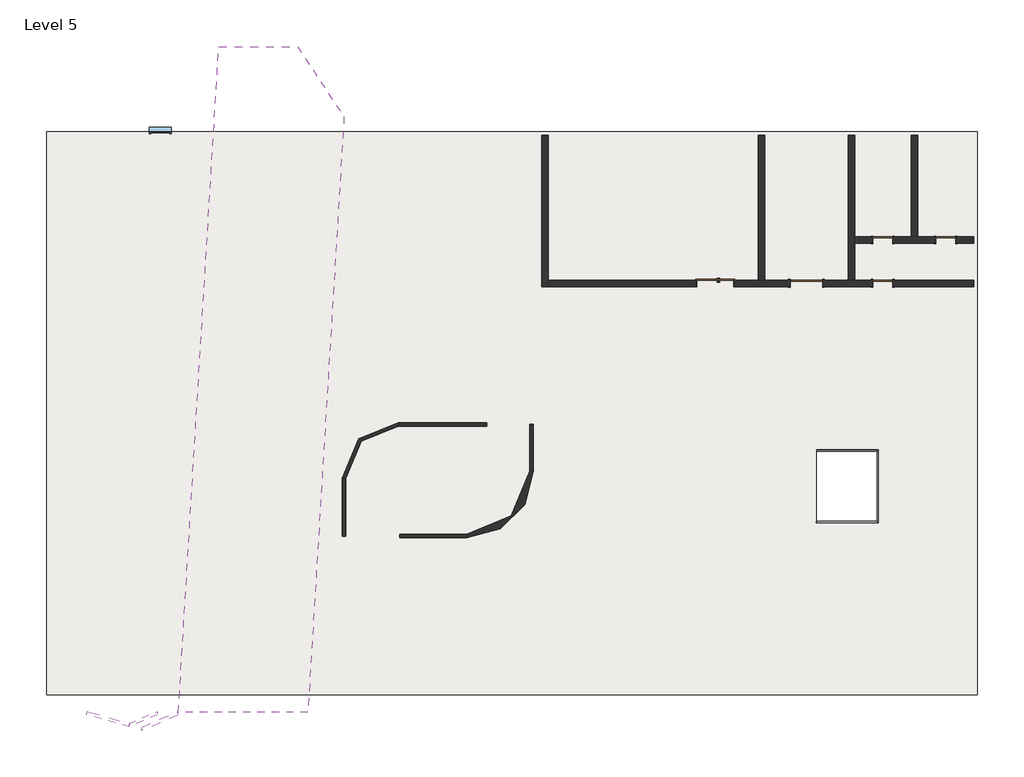
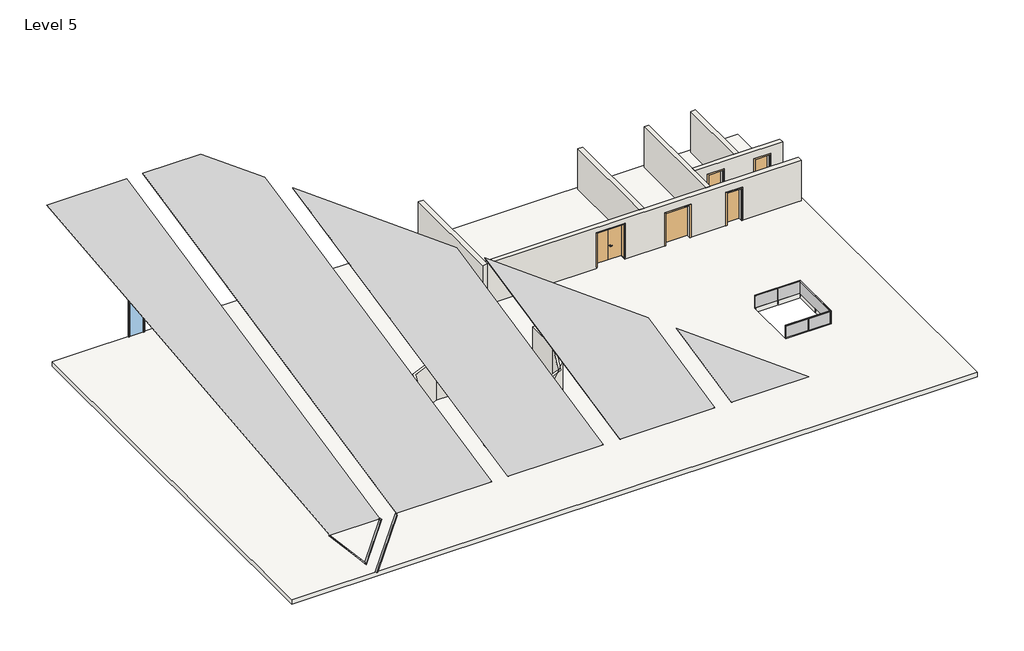
# One storey: 12 walls, 5 doors, 3 members, 1 plate, 1 railing, 1 slab, 1 window.
"""IFC4 building model written with IfcOpenShell, lengths in millimetres."""

import ifcopenshell
import ifcopenshell.guid

model = None  # the IFC model being written
_history = None  # IfcOwnerHistory: only IFC2X3 demands one
_inside = {}  # id of a spatial element -> (the spatial element, [elements in it])
_under = {}  # id of a project, library or spatial element -> (it, [spatial elements below it])
_declared = {}  # id of a project -> (the project, [libraries it declares])
_typed = {}  # id of a type object -> (the type object, [elements of that type])
_made_of = {}  # id of a material, layer set ... -> (it, [elements and type objects made of it])


def new_model(schema):
    """Start an empty IFC model of exactly this schema.

    Asked for "IFC4X3", IfcOpenShell would pick the latest addendum, in which some entities
    have other attributes; the version numbers below select the first issue.
    IFC2X3 requires an IfcOwnerHistory on every rooted entity: one is made here for all.
    """
    global model, _history
    if schema == "IFC4X3":
        model = ifcopenshell.file(schema_version=(4, 3, 0, 0))
    else:
        model = ifcopenshell.file(schema=schema)
    _inside.clear()
    _under.clear()
    _declared.clear()
    _typed.clear()
    _made_of.clear()
    _history = None
    if model.schema == "IFC2X3":
        org = make("IfcOrganization", Name="unknown")
        user = make(
            "IfcPersonAndOrganization",
            ThePerson=make("IfcPerson", FamilyName="unknown"),
            TheOrganization=org,
        )
        app = make(
            "IfcApplication",
            ApplicationDeveloper=org,
            Version="unknown",
            ApplicationFullName="unknown",
            ApplicationIdentifier="unknown",
        )
        _history = make(
            "IfcOwnerHistory",
            OwningUser=user,
            OwningApplication=app,
            ChangeAction="ADDED",
            CreationDate=0,
        )
    return model


def make(cls, **values):
    """One entity of the class cls with the attributes given. An attribute that is None is left unset."""
    return model.create_entity(
        cls, **{name: value for name, value in values.items() if value is not None}
    )


def rooted(cls, **values):
    """An entity with a GlobalId (a new one), such as an element, a storey or a relation."""
    return make(cls, GlobalId=ifcopenshell.guid.new(), OwnerHistory=_history, **values)


def si_unit(unit_type, name, prefix=None):
    """IfcSIUnit, for example si_unit("LENGTHUNIT", "METRE", prefix="MILLI")."""
    return make("IfcSIUnit", UnitType=unit_type, Prefix=prefix, Name=name)


def assignment(units):
    """IfcUnitAssignment: the units of a project."""
    return None if units is None else make("IfcUnitAssignment", Units=units)


def point(xyz):
    """IfcCartesianPoint."""
    return None if xyz is None else make("IfcCartesianPoint", Coordinates=xyz)


def direction(xyz):
    """IfcDirection."""
    return None if xyz is None else make("IfcDirection", DirectionRatios=xyz)


def frame(location, z_axis=None, x_axis=None):
    """IfcAxis2Placement3D, a coordinate frame: its origin and axes. An axis left out is left unset."""
    return make(
        "IfcAxis2Placement3D",
        Location=point(location),
        Axis=direction(z_axis),
        RefDirection=direction(x_axis),
    )


def frame_2d(location, x_axis=None):
    """IfcAxis2Placement2D, a coordinate frame in the plane: its origin and x axis."""
    return make(
        "IfcAxis2Placement2D", Location=point(location), RefDirection=direction(x_axis)
    )


def origin():
    """The frame at (0, 0, 0) with its axes left unset."""
    return frame((0.0, 0.0, 0.0))


def origin_with_axes():
    """The frame at (0, 0, 0) with the z axis (0, 0, 1) and the x axis (1, 0, 0) written out."""
    return frame((0.0, 0.0, 0.0), z_axis=(0.0, 0.0, 1.0), x_axis=(1.0, 0.0, 0.0))


def place(relative_to, where):
    """IfcLocalPlacement: puts the frame where relative to a parent placement (None: the world)."""
    return make(
        "IfcLocalPlacement", PlacementRelTo=relative_to, RelativePlacement=where
    )


def context(
    kind, dimensions, precision=None, world=None, true_north=None, identifier=None
):
    """IfcGeometricRepresentationContext, for example the 3D "Model" context."""
    return make(
        "IfcGeometricRepresentationContext",
        ContextIdentifier=identifier,
        ContextType=kind,
        CoordinateSpaceDimension=dimensions,
        Precision=precision,
        WorldCoordinateSystem=world,
        TrueNorth=true_north,
    )


def project(units=None, contexts=None):
    """IfcProject with its units and contexts."""
    return rooted(
        "IfcProject",
        Name="project",
        RepresentationContexts=contexts,
        UnitsInContext=assignment(units),
    )


def spatial(cls, under=None, at=None, **own):
    """A site, building, storey or space (cls), placed at a placement, below another one or the project."""
    s = rooted(cls, ObjectPlacement=at, **own)
    if under is not None:
        _under.setdefault(under.id(), (under, []))[1].append(s)
    return s


def polyline(points):
    """IfcPolyline through the points."""
    return make("IfcPolyline", Points=[point(p) for p in points])


def circle_curve(where, radius):
    """IfcCircle in the frame where."""
    return make("IfcCircle", Position=where, Radius=radius)


def ellipse_curve(where, semi_axis1, semi_axis2):
    """IfcEllipse in the frame where."""
    return make(
        "IfcEllipse", Position=where, SemiAxis1=semi_axis1, SemiAxis2=semi_axis2
    )


def trimmed(basis, trim1, trim2, sense, master):
    """IfcTrimmedCurve: the piece of a basis curve between two trims."""
    return make(
        "IfcTrimmedCurve",
        BasisCurve=basis,
        Trim1=trim1,
        Trim2=trim2,
        SenseAgreement=sense,
        MasterRepresentation=master,
    )


def segment(curve, same_sense, transition):
    """IfcCompositeCurveSegment."""
    return make(
        "IfcCompositeCurveSegment",
        Transition=transition,
        SameSense=same_sense,
        ParentCurve=curve,
    )


def composite_curve(segments, self_intersect=None):
    """IfcCompositeCurve: segments joined end to end."""
    return make("IfcCompositeCurve", Segments=segments, SelfIntersect=self_intersect)


def outline(outer, holes=None, kind="AREA"):
    """IfcArbitraryClosedProfileDef: a profile drawn as a closed curve; with holes, ...WithVoids."""
    if holes is None:
        return make("IfcArbitraryClosedProfileDef", ProfileType=kind, OuterCurve=outer)
    return make(
        "IfcArbitraryProfileDefWithVoids",
        ProfileType=kind,
        OuterCurve=outer,
        InnerCurves=holes,
    )


def extrude(swept, where, along, depth):
    """IfcExtrudedAreaSolid: the profile swept, set in the frame where, extruded along a direction by depth."""
    return make(
        "IfcExtrudedAreaSolid",
        SweptArea=swept,
        Position=where,
        ExtrudedDirection=direction(along),
        Depth=depth,
    )


def faces_of(points, faces, orient=None, outer=None):
    """IfcFace entities. A face is a list of loops; a loop is a list of indices into points, from 0.

    orient and outer hold one flag for each loop. By default every Orientation is true, the
    first loop of a face is its IfcFaceOuterBound and the others are IfcFaceBound.
    """
    made = []
    for i, loops in enumerate(faces):
        bounds = []
        for j, loop in enumerate(loops):
            is_outer = j == 0 if outer is None else outer[i][j]
            bounds.append(
                make(
                    "IfcFaceOuterBound" if is_outer else "IfcFaceBound",
                    Bound=make("IfcPolyLoop", Polygon=[points[k] for k in loop]),
                    Orientation=True if orient is None else orient[i][j],
                )
            )
        made.append(make("IfcFace", Bounds=bounds))
    return made


def faceted_brep(points, faces, orient=None, outer=None, voids=None):
    """IfcFacetedBrep: a solid bounded by flat faces; with voids (closed shells), ...WithVoids."""
    shared = [point(p) for p in points]
    hull = make("IfcClosedShell", CfsFaces=faces_of(shared, faces, orient, outer))
    if voids is None:
        return make("IfcFacetedBrep", Outer=hull)
    return make(
        "IfcFacetedBrepWithVoids",
        Outer=hull,
        Voids=[
            make(cls, CfsFaces=faces_of(shared, fs, o, b)) for cls, fs, o, b in voids
        ],
    )


def shape(context_of_items, identifier, shape_type, items):
    """IfcShapeRepresentation: the items that make up one representation, for example the "Body"."""
    return make(
        "IfcShapeRepresentation",
        ContextOfItems=context_of_items,
        RepresentationIdentifier=identifier,
        RepresentationType=shape_type,
        Items=items,
    )


def source(mapping_origin, context_of_items, identifier, shape_type, items):
    """IfcRepresentationMap: a shape defined once, which mapped items show again and again."""
    return make(
        "IfcRepresentationMap",
        MappingOrigin=mapping_origin,
        MappedRepresentation=shape(context_of_items, identifier, shape_type, items),
    )


def transform(
    local_origin,
    x_axis=None,
    y_axis=None,
    z_axis=None,
    scale=None,
    scale2=None,
    scale3=None,
    uniform=True,
):
    """IfcCartesianTransformationOperator3D, or its non-uniform kind. x_axis, y_axis, z_axis: its Axis1, 2, 3."""
    if uniform:
        return make(
            "IfcCartesianTransformationOperator3D",
            Axis1=direction(x_axis),
            Axis2=direction(y_axis),
            LocalOrigin=point(local_origin),
            Scale=scale,
            Axis3=direction(z_axis),
        )
    return make(
        "IfcCartesianTransformationOperator3DnonUniform",
        Axis1=direction(x_axis),
        Axis2=direction(y_axis),
        LocalOrigin=point(local_origin),
        Scale=scale,
        Axis3=direction(z_axis),
        Scale2=scale2,
        Scale3=scale3,
    )


def mapped(mapping_source, mapping_target):
    """IfcMappedItem: shows the shape of a source again, moved by a transform."""
    return make(
        "IfcMappedItem", MappingSource=mapping_source, MappingTarget=mapping_target
    )


def made_of(thing, what):
    """Note that an element or type object is made of a material, layer set ...; save() writes the relation."""
    if what is not None:
        _made_of.setdefault(what.id(), (what, []))[1].append(thing)
    return thing


def element(
    cls,
    number,
    at=None,
    inside=None,
    cuts=None,
    type_object=None,
    material=None,
    context=None,
    identifier="Body",
    shape_type=None,
    held_by="IfcProductDefinitionShape",
    body=None,
    shapes=None,
    **own,
):
    """One element of the class cls, such as IfcWall. Its Tag is "e" and its number.

    at: its placement. inside: the storey or other place that contains it. cuts: it is an
    opening in that element (IfcRelVoidsElement). A single representation is given by context,
    identifier, shape_type and body (its items); several are given by shapes. held_by: the class
    of the entity that holds the representations. save() writes the other relations.
    """
    e = rooted(cls, Tag="e%d" % number, ObjectPlacement=at, **own)
    if body is not None:
        shapes = [shape(context, identifier, shape_type, body)]
    if shapes is not None:
        e.Representation = make(held_by, Representations=shapes)
    if inside is not None:
        _inside.setdefault(inside.id(), (inside, []))[1].append(e)
    if cuts is not None:
        rooted(
            "IfcRelVoidsElement", RelatingBuildingElement=cuts, RelatedOpeningElement=e
        )
    if type_object is not None:
        _typed.setdefault(type_object.id(), (type_object, []))[1].append(e)
    return made_of(e, material)


def aggregate(whole, parts):
    """IfcRelAggregates: a whole, such as a stair, and the parts it consists of."""
    return rooted("IfcRelAggregates", RelatingObject=whole, RelatedObjects=parts)


def save(model, path):
    """Write the relations noted so far, then the file.

    IfcRelAggregates (storeys below a building ...), IfcRelContainedInSpatialStructure (elements
    in a storey), IfcRelDefinesByType, IfcRelAssociatesMaterial and IfcRelDeclares: one each for
    every whole, place, type object, material and project.
    """
    for whole, parts in _under.values():
        aggregate(whole, parts)
    for where, things in _inside.values():
        rooted(
            "IfcRelContainedInSpatialStructure",
            RelatedElements=things,
            RelatingStructure=where,
        )
    for kind, things in _typed.values():
        rooted("IfcRelDefinesByType", RelatedObjects=things, RelatingType=kind)
    for what, things in _made_of.values():
        rooted("IfcRelAssociatesMaterial", RelatedObjects=things, RelatingMaterial=what)
    for by, libraries in _declared.values():
        rooted("IfcRelDeclares", RelatingContext=by, RelatedDefinitions=libraries)
    model.write(path)


def plane_surface(at):
    """IfcPlane: the flat surface through the origin of the frame at, square to its z axis."""
    return make("IfcPlane", Position=at)


def cylinder_surface(at, radius):
    """IfcCylindricalSurface: all points at the distance radius from the z axis of the frame at."""
    return make("IfcCylindricalSurface", Position=at, Radius=radius)


def advanced_brep(points, edges, surfaces, faces):
    """IfcAdvancedBrep: a solid bounded by faces that lie on surfaces and meet in shared edges.

    An edge is (start, end): straight between two places in points (the first is 0);
    or (start, end, curve); or (start, end, curve, False) where it runs against its curve.
    A face is (place in surfaces, loops), or (place, loops, False) where it looks against
    its surface's normal. A loop lists edges by number (the first is 1), with a minus sign
    where the edge is run from its end to its start. The first loop is the outer one.
    """
    corners = [point(p) for p in points]
    vertices = [make("IfcVertexPoint", VertexGeometry=c) for c in corners]
    made = []
    for start, end, *more in edges:
        made.append(
            make(
                "IfcEdgeCurve",
                EdgeStart=vertices[start],
                EdgeEnd=vertices[end],
                EdgeGeometry=more[0] if more else make("IfcPolyline", Points=[corners[start], corners[end]]),
                SameSense=more[1] if len(more) > 1 else True,
            )
        )
    hull = []
    for where, loops, *sense in faces:
        bounds = []
        for j, loop in enumerate(loops):
            ring = [make("IfcOrientedEdge", EdgeElement=made[abs(k) - 1], Orientation=k > 0) for k in loop]
            bounds.append(
                make(
                    "IfcFaceOuterBound" if j == 0 else "IfcFaceBound",
                    Bound=make("IfcEdgeLoop", EdgeList=ring),
                    Orientation=True,
                )
            )
        hull.append(make("IfcAdvancedFace", Bounds=bounds, FaceSurface=surfaces[where], SameSense=sense[0] if sense else True))
    return make("IfcAdvancedBrep", Outer=make("IfcClosedShell", CfsFaces=hull))


def door_double_flush_variable_door_double_flush_variable_ac6c3b87(model_context):
    return source(origin(), model_context, "Body", "SolidModel", [
        advanced_brep(
        [(90.0, 139.4346141, 1000.0), (110.0, 139.4346141, 1000.0), (90.0, 69.4346141, 1000.0), (110.0, 89.4346141, 1000.0), (220.0, 69.4346141, 1000.0), (220.0, 89.4346141, 1000.0)],
        [
            (0, 1, circle_curve(frame((100.0, 139.4346141, 1000.0), z_axis=(0.0, 1.0, 0.0), x_axis=(1.0, 0.0, 0.0)), 10.0)),
            (1, 0, circle_curve(frame((100.0, 139.4346141, 1000.0), z_axis=(0.0, 1.0, 0.0), x_axis=(1.0, 0.0, 0.0)), 10.0)),
            (0, 2),
            (2, 3, ellipse_curve(frame((100.0, 79.4346141, 1000.0), z_axis=(-0.7071067811865385, 0.7071067811865565, 0.0), x_axis=(0.7071067811865563, 0.7071067811865386, 0.0)), 14.1421356, 10.0)),
            (3, 1),
            (3, 2, ellipse_curve(frame((100.0, 79.4346141, 1000.0), z_axis=(-0.7071067811865385, 0.7071067811865565, 0.0), x_axis=(0.7071067811865563, 0.7071067811865386, 0.0)), 14.1421356, 10.0)),
            (4, 5, circle_curve(frame((220.0, 79.4346141, 1000.0), z_axis=(1.0, 0.0, 0.0), x_axis=(0.0, 1.0, 0.0)), 10.0)),
            (5, 4, circle_curve(frame((220.0, 79.4346141, 1000.0), z_axis=(1.0, 0.0, 0.0), x_axis=(0.0, 1.0, 0.0)), 10.0)),
            (2, 4),
            (5, 3),
        ],
        [
            plane_surface(frame((100.0, 139.4346141, -287.7526403), z_axis=(0.0, 1.0, 0.0), x_axis=(0.0, 0.0, 1.0))),
            cylinder_surface(frame((100.0, 139.4346141, 1000.0), z_axis=(0.0, 1.0, 0.0), x_axis=(1.0, 0.0, 0.0)), 10.0),
            plane_surface(frame((220.0, 79.4346141, -287.7526403), z_axis=(1.0, 0.0, 0.0), x_axis=(0.0, 0.0, 1.0))),
            cylinder_surface(frame((100.0, 79.4346141, 1000.0), z_axis=(-1.0, 0.0, 0.0), x_axis=(0.0, 1.0, 0.0)), 10.0),
        ],
        [
            (0, [[1, 2]]),
            (1, [[-1, 3, 4, 5]]),
            (1, [[-2, -5, 6, -3]]),
            (2, [[7, 8]]),
            (3, [[-4, 9, -8, 10]]),
            (3, [[-6, -10, -7, -9]]),
        ],
    ),
        advanced_brep(
        [(110.0, 199.4346141, 1000.0), (90.0, 199.4346141, 1000.0), (110.0, 229.4346141, 1000.0), (90.0, 249.4346141, 1000.0), (220.0, 229.4346141, 1000.0), (220.0, 249.4346141, 1000.0)],
        [
            (0, 1, circle_curve(frame((100.0, 199.4346141, 1000.0), z_axis=(0.0, -1.0, 0.0), x_axis=(-1.0, 0.0, 0.0)), 10.0)),
            (1, 0, circle_curve(frame((100.0, 199.4346141, 1000.0), z_axis=(0.0, -1.0, 0.0), x_axis=(-1.0, 0.0, 0.0)), 10.0)),
            (0, 2),
            (2, 3, ellipse_curve(frame((100.0, 239.4346141, 1000.0), z_axis=(-0.7071067811865475, -0.7071067811865475, 0.0), x_axis=(0.7071067811865474, -0.7071067811865476, 0.0)), 14.1421356, 10.0)),
            (3, 1),
            (3, 2, ellipse_curve(frame((100.0, 239.4346141, 1000.0), z_axis=(-0.7071067811865475, -0.7071067811865475, 0.0), x_axis=(0.7071067811865474, -0.7071067811865476, 0.0)), 14.1421356, 10.0)),
            (4, 5, circle_curve(frame((220.0, 239.4346141, 1000.0), z_axis=(1.0, 0.0, 0.0), x_axis=(0.0, 1.0, 0.0)), 10.0)),
            (5, 4, circle_curve(frame((220.0, 239.4346141, 1000.0), z_axis=(1.0, 0.0, 0.0), x_axis=(0.0, 1.0, 0.0)), 10.0)),
            (2, 4),
            (5, 3),
        ],
        [
            plane_surface(frame((100.0, 199.4346141, -287.7526403), z_axis=(0.0, -1.0, 0.0), x_axis=(0.0, 0.0, 1.0))),
            cylinder_surface(frame((100.0, 199.4346141, 1000.0), z_axis=(0.0, -1.0, 0.0), x_axis=(-1.0, 0.0, 0.0)), 10.0),
            plane_surface(frame((220.0, 239.4346141, -287.7526403), z_axis=(1.0, 0.0, 0.0), x_axis=(0.0, 0.0, 1.0))),
            cylinder_surface(frame((100.0, 239.4346141, 1000.0), z_axis=(-1.0, 0.0, 0.0), x_axis=(0.0, 1.0, 0.0)), 10.0),
        ],
        [
            (0, [[1, 2]]),
            (1, [[-1, 3, 4, 5]]),
            (1, [[-2, -5, 6, -3]]),
            (2, [[7, 8]]),
            (3, [[-4, 9, -8, 10]]),
            (3, [[-6, -10, -7, -9]]),
        ],
    ),
        extrude(outline(composite_curve([segment(trimmed(circle_curve(frame_2d((1000.0, 100.0)), 20.0), [point((1000.0, 80.0))], [point((1000.0, 120.0))], False, "CARTESIAN"), True, "CONTINUOUS"), segment(trimmed(circle_curve(frame_2d((1000.0, 100.0)), 20.0), [point((1000.0, 120.0))], [point((1000.0, 80.0))], False, "CARTESIAN"), True, "CONTINUOUS")], self_intersect=False)), frame((0.0, 129.4346141, 0.0), z_axis=(0.0, 1.0, 0.0), x_axis=(0.0, 0.0, 1.0)), (0.0, 0.0, 1.0), 10.0),
        extrude(outline(composite_curve([segment(trimmed(circle_curve(frame_2d((1000.0, 100.0)), 20.0), [point((1000.0, 80.0))], [point((1000.0, 120.0))], False, "CARTESIAN"), True, "CONTINUOUS"), segment(trimmed(circle_curve(frame_2d((1000.0, 100.0)), 20.0), [point((1000.0, 120.0))], [point((1000.0, 80.0))], False, "CARTESIAN"), True, "CONTINUOUS")], self_intersect=False)), frame((0.0, 189.4346141, 0.0), z_axis=(0.0, 1.0, 0.0), x_axis=(0.0, 0.0, 1.0)), (0.0, 0.0, 1.0), 10.0),
        extrude(outline(polyline([(0.0, 164.4346141), (-871.25, 164.4346141), (-871.25, 189.4346141), (0.0, 189.4346141), (0.0, 164.4346141)])), frame((0.0, 0.0, 100.0), z_axis=(0.0, 0.0, 1.0), x_axis=(1.0, 0.0, 0.0)), (0.0, 0.0, 1.0), 2250.0),
        extrude(outline(polyline([(871.25, 164.4346141), (0.0, 164.4346141), (0.0, 189.4346141), (871.25, 189.4346141), (871.25, 164.4346141)])), frame((0.0, 0.0, 100.0), z_axis=(0.0, 0.0, 1.0), x_axis=(1.0, 0.0, 0.0)), (0.0, 0.0, 1.0), 2250.0),
        faceted_brep([(905.75, -150.5653859, 100.0), (856.25, -150.5653859, 100.0), (856.25, 164.4346141, 100.0), (871.25, 164.4346141, 100.0), (871.25, 189.4346141, 100.0), (905.75, 189.4346141, 100.0), (905.75, 164.4346141, 100.0), (900.75, 164.4346141, 100.0), (900.75, 184.4346141, 100.0), (876.25, 184.4346141, 100.0), (876.25, 159.4346141, 100.0), (861.25, 159.4346141, 100.0), (861.25, -145.5653859, 100.0), (900.75, -145.5653859, 100.0), (900.75, -135.5653859, 100.0), (905.75, -135.5653859, 100.0), (905.75, -150.5653859, 2384.5), (-905.75, -150.5653859, 2384.5), (-905.75, -150.5653859, 100.0), (-856.25, -150.5653859, 100.0), (-856.25, -150.5653859, 2335.0), (856.25, -150.5653859, 2335.0), (856.25, 164.4346141, 2335.0), (-856.25, 164.4346141, 2335.0), (-856.25, 164.4346141, 100.0), (-871.25, 164.4346141, 100.0), (-871.25, 164.4346141, 2350.0), (871.25, 164.4346141, 2350.0), (871.25, 189.4346141, 2350.0), (-871.25, 189.4346141, 2350.0), (-871.25, 189.4346141, 100.0), (-905.75, 189.4346141, 100.0), (-905.75, 189.4346141, 2384.5), (905.75, 189.4346141, 2384.5), (905.75, 164.4346141, 2384.5), (-905.75, 164.4346141, 2384.5), (-905.75, 164.4346141, 100.0), (-900.75, 164.4346141, 100.0), (-900.75, 164.4346141, 2379.5), (900.75, 164.4346141, 2379.5), (900.75, 184.4346141, 2379.5), (-900.75, 184.4346141, 2379.5), (-900.75, 184.4346141, 100.0), (-876.25, 184.4346141, 100.0), (-876.25, 184.4346141, 2355.0), (876.25, 184.4346141, 2355.0), (876.25, 159.4346141, 2355.0), (-876.25, 159.4346141, 2355.0), (-876.25, 159.4346141, 100.0), (-861.25, 159.4346141, 100.0), (-861.25, 159.4346141, 2340.0), (861.25, 159.4346141, 2340.0), (861.25, -145.5653859, 2340.0), (-861.25, -145.5653859, 2340.0), (-861.25, -145.5653859, 100.0), (-900.75, -145.5653859, 100.0), (-900.75, -145.5653859, 2379.5), (900.75, -145.5653859, 2379.5), (900.75, -135.5653859, 2379.5), (-900.75, -135.5653859, 2379.5), (-900.75, -135.5653859, 100.0), (-905.75, -135.5653859, 100.0), (-905.75, -135.5653859, 2384.5), (905.75, -135.5653859, 2384.5)], [[[0, 1, 2, 3, 4, 5, 6, 7, 8, 9, 10, 11, 12, 13, 14, 15]], [[1, 0, 16, 17, 18, 19, 20, 21]], [[2, 1, 21, 22]], [[3, 2, 22, 23, 24, 25, 26, 27]], [[4, 3, 27, 28]], [[5, 4, 28, 29, 30, 31, 32, 33]], [[6, 5, 33, 34]], [[7, 6, 34, 35, 36, 37, 38, 39]], [[8, 7, 39, 40]], [[9, 8, 40, 41, 42, 43, 44, 45]], [[10, 9, 45, 46]], [[11, 10, 46, 47, 48, 49, 50, 51]], [[12, 11, 51, 52]], [[13, 12, 52, 53, 54, 55, 56, 57]], [[14, 13, 57, 58]], [[15, 14, 58, 59, 60, 61, 62, 63]], [[0, 15, 63, 16]], [[17, 62, 61, 18]], [[18, 61, 60, 55, 54, 49, 48, 43, 42, 37, 36, 31, 30, 25, 24, 19]], [[23, 20, 19, 24]], [[29, 26, 25, 30]], [[35, 32, 31, 36]], [[41, 38, 37, 42]], [[47, 44, 43, 48]], [[53, 50, 49, 54]], [[59, 56, 55, 60]], [[22, 21, 20, 23]], [[28, 27, 26, 29]], [[34, 33, 32, 35]], [[40, 39, 38, 41]], [[46, 45, 44, 47]], [[52, 51, 50, 53]], [[58, 57, 56, 59]], [[16, 63, 62, 17]]]),
    ])


def m_single_flush_0915_x_2134mm_1c84716f(model_context):
    return source(origin(), model_context, "Body", "SweptSolid", [
        extrude(outline(polyline([(2210.0, -533.5), (0.0, -533.5), (0.0, -457.5), (2134.0, -457.5), (2134.0, 457.5), (0.0, 457.5), (0.0, 533.5), (2210.0, 533.5), (2210.0, -533.5)])), frame((0.0, -175.0, 0.0), z_axis=(0.0, 1.0, 0.0), x_axis=(0.0, 0.0, 1.0)), (0.0, 0.0, 1.0), 25.0),
        extrude(outline(polyline([(2210.0, 533.5), (2210.0, -533.5), (0.0, -533.5), (0.0, -457.5), (2134.0, -457.5), (2134.0, 457.5), (0.0, 457.5), (0.0, 533.5), (2210.0, 533.5)])), frame((0.0, 150.0, 0.0), z_axis=(0.0, 1.0, 0.0), x_axis=(0.0, 0.0, 1.0)), (0.0, 0.0, 1.0), 25.0),
        extrude(outline(polyline([(457.5, -99.0), (457.5, -150.0), (-457.5, -150.0), (-457.5, -99.0), (457.5, -99.0)])), origin_with_axes(), (0.0, 0.0, 1.0), 2134.0),
    ])


def m_single_flush_1500_x_2134mm_2_edebd810(model_context):
    return source(origin(), model_context, "Body", "SweptSolid", [
        extrude(outline(polyline([(2210.0, -826.0), (0.0, -826.0), (0.0, -750.0), (2134.0, -750.0), (2134.0, 750.0), (0.0, 750.0), (0.0, 826.0), (2210.0, 826.0), (2210.0, -826.0)])), frame((0.0, -175.0, 0.0), z_axis=(0.0, 1.0, 0.0), x_axis=(0.0, 0.0, 1.0)), (0.0, 0.0, 1.0), 25.0),
        extrude(outline(polyline([(2210.0, 826.0), (2210.0, -826.0), (0.0, -826.0), (0.0, -750.0), (2134.0, -750.0), (2134.0, 750.0), (0.0, 750.0), (0.0, 826.0), (2210.0, 826.0)])), frame((0.0, 150.0, 0.0), z_axis=(0.0, 1.0, 0.0), x_axis=(0.0, 0.0, 1.0)), (0.0, 0.0, 1.0), 25.0),
        extrude(outline(polyline([(750.0, -99.0), (750.0, -150.0), (-750.0, -150.0), (-750.0, -99.0), (750.0, -99.0)])), origin_with_axes(), (0.0, 0.0, 1.0), 2134.0),
    ])


def rectangular_mullion_50_x_150mm_faae0562(model_context):
    return source(origin(), model_context, "Body", "SweptSolid", [
        extrude(outline(polyline([(0.0, 0.0), (-85.321119, -50.0), (-2553.6011295, -50.0), (-2625.2230034, 0.0), (0.0, 0.0)])), frame((0.0, -75.0, 0.0), z_axis=(0.0, 1.0, 0.0), x_axis=(0.0, 0.0, 1.0)), (0.0, 0.0, 1.0), 150.0),
    ])


def rectangular_mullion_50_x_150mm_82bd072a(model_context):
    return source(origin(), model_context, "Body", "SweptSolid", [
        extrude(outline(polyline([(0.0, 0.0), (-34.9055374, -50.0), (-3342.3079561, -50.0), (-3371.6090252, 0.0), (0.0, 0.0)])), frame((0.0, -75.0, 0.0), z_axis=(0.0, 1.0, 0.0), x_axis=(0.0, 0.0, 1.0)), (0.0, 0.0, 1.0), 150.0),
    ])


def rectangular_mullion_50_x_150mm_a1351d1e(model_context):
    return source(origin(), model_context, "Body", "SweptSolid", [
        extrude(outline(polyline([(0.0, 0.0), (-71.6218739, -50.0), (-2906.9650483, -50.0), (-3015.6254931, 0.0), (0.0, 0.0)])), frame((0.0, -75.0, 0.0), z_axis=(0.0, 1.0, 0.0), x_axis=(0.0, 0.0, 1.0)), (0.0, 0.0, 1.0), 150.0),
    ])


def system_panel_perforated_metal_panel_mpk_dbcede24(model_context):
    return source(origin(), model_context, "Body", "SweptSolid", [
        extrude(outline(polyline([(2659.2774582, 8492.4699444), (0.0, 12533.2512196), (8060.1335901, 12533.2512196), (2659.2774582, 8492.4699444)])), frame((0.0, 0.0, 0.0), z_axis=(0.0, 1.0, 0.0), x_axis=(0.0, 0.0, 1.0)), (0.0, 0.0, 1.0), 20.0),
        extrude(outline(polyline([(16496.5090545, -12533.2512196), (14766.0852816, -9903.8663249), (39552.7658936, 8640.8888851), (42308.3486088, 4453.7714396), (16496.5090545, -12533.2512196)])), frame((0.0, 0.0, 0.0), z_axis=(0.0, 1.0, 0.0), x_axis=(0.0, 0.0, 1.0)), (0.0, 0.0, 1.0), 20.0),
        extrude(outline(polyline([(14203.8559644, -9049.5569371), (10917.8924462, -4056.524031), (33091.572061, 12533.2512196), (36991.1643838, 12533.2512196), (38990.5365764, 9495.1982729), (14203.8559644, -9049.5569371)])), frame((0.0, 0.0, 0.0), z_axis=(0.0, 1.0, 0.0), x_axis=(0.0, 0.0, 1.0)), (0.0, 0.0, 1.0), 20.0),
        extrude(outline(polyline([(10355.663129, -3202.2146433), (7069.6996108, 1790.8182628), (21427.8969383, 12533.2512196), (31387.4838355, 12533.2512196), (10355.663129, -3202.2146433)])), frame((0.0, 0.0, 0.0), z_axis=(0.0, 1.0, 0.0), x_axis=(0.0, 0.0, 1.0)), (0.0, 0.0, 1.0), 20.0),
        extrude(outline(polyline([(6507.4702936, 2645.1276506), (3221.5067754, 7638.1605567), (9764.2218156, 12533.2512196), (19723.8087128, 12533.2512196), (6507.4702936, 2645.1276506)])), frame((0.0, 0.0, 0.0), z_axis=(0.0, 1.0, 0.0), x_axis=(0.0, 0.0, 1.0)), (0.0, 0.0, 1.0), 20.0),
    ])


def glas_mpk_389492d2(model_context):
    return source(origin(), model_context, "Body", "SolidModel", [
        faceted_brep([(28820.4268037, 1294.9571597, 12843.2628643), (28820.4268037, 1244.9571597, 12843.2628643), (28820.4268037, 1244.9571597, 12856.7371357), (28820.4268037, 1294.9571597, 12856.7371357), (31660.4268037, 1294.9571597, 12843.2628643), (31610.4268037, 1244.9571597, 12843.2628643), (31610.4268037, 1244.9571597, 12856.7371357), (31660.4268037, 1294.9571597, 12856.7371357), (31660.4268037, -2045.7721864, 12843.2628643), (31610.4268037, -1995.7721864, 12843.2628643), (31610.4268037, -1995.7721864, 12856.7371357), (31660.4268037, -2045.7721864, 12856.7371357), (28820.4268037, -2045.7721864, 12843.2628643), (28820.4268037, -2045.7721864, 12856.7371357), (28820.4268037, -1995.7721864, 12856.7371357), (28820.4268037, -1995.7721864, 12843.2628643)], [[[0, 1, 2, 3]], [[1, 0, 4, 5]], [[2, 1, 5, 6]], [[3, 2, 6, 7]], [[0, 3, 7, 4]], [[5, 4, 8, 9]], [[6, 5, 9, 10]], [[7, 6, 10, 11]], [[4, 7, 11, 8]], [[12, 13, 14, 15]], [[9, 8, 12, 15]], [[10, 9, 15, 14]], [[11, 10, 14, 13]], [[8, 11, 13, 12]]]),
        faceted_brep([(28820.4268037, 1254.9571597, 12842.8769824), (28820.4268037, 1269.1492837, 12842.8769824), (28820.4268037, 1269.1492837, 12042.8769824), (28820.4268037, 1254.9571597, 12042.8769824), (31620.4268037, 1254.9571597, 12842.8769824), (31634.6189277, 1269.1492837, 12842.8769824), (31634.6189277, 1269.1492837, 12042.8769824), (31620.4268037, 1254.9571597, 12042.8769824), (31620.4268037, -2005.7721864, 12842.8769824), (31634.6189277, -2019.9643104, 12842.8769824), (31634.6189277, -2019.9643104, 12042.8769824), (31620.4268037, -2005.7721864, 12042.8769824), (28820.4268037, -2005.7721864, 12842.8769824), (28820.4268037, -2005.7721864, 12042.8769824), (28820.4268037, -2019.9643104, 12042.8769824), (28820.4268037, -2019.9643104, 12842.8769824)], [[[0, 1, 2, 3]], [[1, 0, 4, 5]], [[2, 1, 5, 6]], [[3, 2, 6, 7]], [[0, 3, 7, 4]], [[5, 4, 8, 9]], [[6, 5, 9, 10]], [[7, 6, 10, 11]], [[4, 7, 11, 8]], [[12, 13, 14, 15]], [[9, 8, 12, 15]], [[10, 9, 15, 14]], [[11, 10, 14, 13]], [[8, 11, 13, 12]]]),
        extrude(outline(polyline([(30251.6768037, -2020.7721864), (30251.6768037, -2045.7721864), (30226.6768037, -2045.7721864), (30226.6768037, -2020.7721864), (30251.6768037, -2020.7721864)])), frame((0.0, 0.0, 11800.0), z_axis=(0.0, 0.0, 1.0), x_axis=(1.0, 0.0, 0.0)), (0.0, 0.0, 1.0), 1043.2628643),
        extrude(outline(polyline([(31635.4268037, -362.9075133), (31660.4268037, -362.9075133), (31660.4268037, -387.9075133), (31635.4268037, -387.9075133), (31635.4268037, -362.9075133)])), frame((0.0, 0.0, 11800.0), z_axis=(0.0, 0.0, 1.0), x_axis=(1.0, 0.0, 0.0)), (0.0, 0.0, 1.0), 1043.2628643),
        extrude(outline(polyline([(30226.6768037, 1269.9571597), (30226.6768037, 1294.9571597), (30251.6768037, 1294.9571597), (30251.6768037, 1269.9571597), (30226.6768037, 1269.9571597)])), frame((0.0, 0.0, 11800.0), z_axis=(0.0, 0.0, 1.0), x_axis=(1.0, 0.0, 0.0)), (0.0, 0.0, 1.0), 1043.2628643),
        extrude(outline(polyline([(31635.4268037, -2030.7721864), (31660.4268037, -2030.7721864), (31660.4268037, -2055.7721864), (31635.4268037, -2055.7721864), (31635.4268037, -2030.7721864)])), frame((0.0, 0.0, 11800.0), z_axis=(0.0, 0.0, 1.0), x_axis=(1.0, 0.0, 0.0)), (0.0, 0.0, 1.0), 1043.2628643),
        extrude(outline(polyline([(31645.4268037, 1269.9571597), (31645.4268037, 1294.9571597), (31670.4268037, 1294.9571597), (31670.4268037, 1269.9571597), (31645.4268037, 1269.9571597)])), frame((0.0, 0.0, 11800.0), z_axis=(0.0, 0.0, 1.0), x_axis=(1.0, 0.0, 0.0)), (0.0, 0.0, 1.0), 1043.2628643),
        extrude(outline(polyline([(28832.9268037, -2020.7721864), (28832.9268037, -2045.7721864), (28807.9268037, -2045.7721864), (28807.9268037, -2020.7721864), (28832.9268037, -2020.7721864)])), frame((0.0, 0.0, 11800.0), z_axis=(0.0, 0.0, 1.0), x_axis=(1.0, 0.0, 0.0)), (0.0, 0.0, 1.0), 1043.2628643),
        extrude(outline(polyline([(28820.4268037, 1269.9571597), (28820.4268037, 1294.9571597), (28845.4268037, 1294.9571597), (28845.4268037, 1269.9571597), (28820.4268037, 1269.9571597)])), frame((0.0, 0.0, 11800.0), z_axis=(0.0, 0.0, 1.0), x_axis=(1.0, 0.0, 0.0)), (0.0, 0.0, 1.0), 1043.2628643),
    ])


def window_variable_standard_5cf830ff(model_context):
    return source(origin(), model_context, "Body", "SolidModel", [
        extrude(outline(polyline([(9000.0, 500.0), (9000.0, -500.0), (1000.0, -500.0), (1000.0, 500.0), (9000.0, 500.0)]), holes=[polyline([(8920.0, 440.0), (1080.0, 440.0), (1080.0, -440.0), (8920.0, -440.0), (8920.0, 440.0)])]), frame((0.0, 35.0, 0.0), z_axis=(0.0, 1.0, 0.0), x_axis=(0.0, 0.0, 1.0)), (0.0, 0.0, 1.0), 60.0),
        faceted_brep([(470.0, 35.0, 8950.0), (470.0, 5.0, 8950.0), (470.0, 5.0, 1050.0), (470.0, 35.0, 1050.0), (-470.0, 5.0, 8950.0), (-470.0, 5.0, 1050.0), (410.0, 5.0, 1110.0), (-410.0, 5.0, 1110.0), (-410.0, 5.0, 8890.0), (410.0, 5.0, 8890.0), (-470.0, 35.0, 1050.0), (-470.0, 35.0, 8950.0), (440.0, 35.0, 8920.0), (-440.0, 35.0, 8920.0), (-440.0, 35.0, 1080.0), (440.0, 35.0, 1080.0), (440.0, 65.0, 8920.0), (440.0, 65.0, 1080.0), (-440.0, 65.0, 1080.0), (-440.0, 65.0, 8920.0), (410.0, 65.0, 8890.0), (-410.0, 65.0, 8890.0), (-410.0, 65.0, 1110.0), (410.0, 65.0, 1110.0)], [[[0, 1, 2, 3]], [[1, 4, 5, 2], [6, 7, 8, 9]], [[3, 2, 5, 10]], [[3, 10, 11, 0], [12, 13, 14, 15]], [[16, 12, 15, 17]], [[17, 15, 14, 18]], [[17, 18, 19, 16], [20, 21, 22, 23]], [[9, 20, 23, 6]], [[6, 23, 22, 7]], [[10, 5, 4, 11]], [[18, 14, 13, 19]], [[7, 22, 21, 8]], [[11, 4, 1, 0]], [[19, 13, 12, 16]], [[8, 21, 20, 9]]]),
        extrude(outline(polyline([(-500.0, -205.0), (-500.0, 35.0), (500.0, 35.0), (500.0, -205.0), (-500.0, -205.0)])), frame((0.0, 0.0, 1005.0), z_axis=(0.0, 0.0, 1.0), x_axis=(1.0, 0.0, 0.0)), (0.0, 0.0, 1.0), 15.0),
        extrude(outline(polyline([(105.0221543, 1020.0), (205.0, 1000.0), (205.0, 990.0), (203.0, 990.0), (203.0, 998.3604634), (104.8240723, 1018.0), (95.0, 1018.0), (95.0, 1020.0), (105.0221543, 1020.0)])), frame((-500.0, 0.0, 0.0), z_axis=(1.0, 0.0, 0.0), x_axis=(0.0, 1.0, 0.0)), (0.0, 0.0, 1.0), 1000.0),
        extrude(outline(polyline([(410.0, 20.0), (-410.0, 20.0), (-410.0, 50.0), (410.0, 50.0), (410.0, 20.0)])), frame((0.0, 0.0, 1110.0), z_axis=(0.0, 0.0, 1.0), x_axis=(1.0, 0.0, 0.0)), (0.0, 0.0, 1.0), 7780.0),
    ])


model = new_model("IFC4")

# Units and contexts
model_context = context("Model", 3, world=origin())
ifc_project = project(units=[si_unit("LENGTHUNIT", "METRE", prefix="MILLI")], contexts=[model_context])

# Site, building, storey
site = spatial("IfcSite", under=ifc_project)
building = spatial("IfcBuilding", under=site)
storey = spatial("IfcBuildingStorey", under=building, Name="Level 5", Elevation=12000.0)

# Doors
placement = place(None, origin())
door_double_flush_variable_door_double_flush_variable_shape = door_double_flush_variable_door_double_flush_variable_ac6c3b87(model_context)
element("IfcDoor", 1, ObjectType="Door Double Flush - Variable : Door Double Flush - Variable", at=placement, inside=storey, context=model_context, shape_type="MappedRepresentation", body=[
    mapped(door_double_flush_variable_door_double_flush_variable_shape, transform((24136.7471367, 8984.3231089, 12000.0), x_axis=(1.0, 0.0, 0.0), y_axis=(0.0, 1.0, 0.0), z_axis=(0.0, 0.0, 1.0))),
])
m_single_flush_0915_x_2134mm_shape = m_single_flush_0915_x_2134mm_1c84716f(model_context)
element("IfcDoor", 2, ObjectType="M_Single-Flush : 0915 x 2134mm", at=placement, inside=storey, context=model_context, shape_type="MappedRepresentation", body=[
    mapped(m_single_flush_0915_x_2134mm_shape, transform((34787.1221367, 10998.757723, 12000.0), x_axis=(-1.0, 0.0, 0.0), y_axis=(0.0, -1.0, 0.0), z_axis=(0.0, 0.0, 1.0))),
])
element("IfcDoor", 3, ObjectType="M_Single-Flush : 0915 x 2134mm", at=placement, inside=storey, context=model_context, shape_type="MappedRepresentation", body=[
    mapped(m_single_flush_0915_x_2134mm_shape, transform((31874.3721367, 10998.757723, 12000.0), x_axis=(-1.0, 0.0, 0.0), y_axis=(0.0, -1.0, 0.0), z_axis=(0.0, 0.0, 1.0))),
])
element("IfcDoor", 4, ObjectType="M_Single-Flush : 0915 x 2134mm", at=placement, inside=storey, context=model_context, shape_type="MappedRepresentation", body=[
    mapped(m_single_flush_0915_x_2134mm_shape, transform((31874.3721367, 8998.757723, 12000.0), x_axis=(-1.0, 0.0, 0.0), y_axis=(0.0, -1.0, 0.0), z_axis=(0.0, 0.0, 1.0))),
])
m_single_flush_1500_x_2134mm_2_shape = m_single_flush_1500_x_2134mm_2_edebd810(model_context)
element("IfcDoor", 5, ObjectType="M_Single-Flush : 1500 x 2134mm 2", at=placement, inside=storey, context=model_context, shape_type="MappedRepresentation", body=[
    mapped(m_single_flush_1500_x_2134mm_2_shape, transform((28342.9971367, 8998.757723, 12000.0), x_axis=(-1.0, 0.0, 0.0), y_axis=(0.0, -1.0, 0.0), z_axis=(0.0, 0.0, 1.0))),
])

# Members
rectangular_mullion_50_x_150mm_shape = rectangular_mullion_50_x_150mm_faae0562(model_context)
element("IfcMember", 6, ObjectType="Rectangular Mullion : 50 x 150mm", at=placement, inside=storey, context=model_context, shape_type="MappedRepresentation", body=[
    mapped(rectangular_mullion_50_x_150mm_shape, transform((-1622.1158471, -10856.2576342, 16077.9460567), x_axis=(0.8724314351462177, -0.1182360666014563, -0.4742189615813852), y_axis=(0.0, 0.9702957262759963, -0.24192189559966853), z_axis=(0.4887365251019319, 0.21106026657131113, 0.8465164929912092))),
])
rectangular_mullion_50_x_150mm_2_shape = rectangular_mullion_50_x_150mm_82bd072a(model_context)
element("IfcMember", 7, ObjectType="Rectangular Mullion : 50 x 150mm", at=placement, inside=storey, context=model_context, shape_type="MappedRepresentation", body=[
    mapped(rectangular_mullion_50_x_150mm_2_shape, transform((-2347.4110859, -11567.8703339, 13223.823409), x_axis=(-0.8724314351462177, 0.11823606660145629, 0.47421896158138516), y_axis=(0.0, 0.9702957262759963, -0.2419218955996686), z_axis=(-0.48873652510193183, -0.2110602665713112, -0.8465164929912092))),
])
rectangular_mullion_50_x_150mm_3_shape = rectangular_mullion_50_x_150mm_a1351d1e(model_context)
element("IfcMember", 8, ObjectType="Rectangular Mullion : 50 x 150mm", at=placement, inside=storey, context=model_context, shape_type="MappedRepresentation", body=[
    mapped(rectangular_mullion_50_x_150mm_3_shape, transform((-2905.1582154, -11410.3379011, 13855.6514866), x_axis=(-0.7594865733990558, -0.15737575195413053, -0.6311996653384985), y_axis=(0.0, 0.9702957262759964, -0.24192189559966842), z_axis=(0.6505229779389508, -0.1837364315191978, -0.7369265763331043))),
])

# Plate
system_panel_perforated_metal_panel_mpk_shape = system_panel_perforated_metal_panel_mpk_dbcede24(model_context)
element("IfcPlate", 9, ObjectType="System Panel : Perforated Metal Panel - MPK", at=placement, inside=storey, context=model_context, shape_type="MappedRepresentation", body=[
    mapped(system_panel_perforated_metal_panel_mpk_shape, transform((14721.3878068, -17658.8396177, 15362.9658795), x_axis=(0.83533461340766, 0.5467302903451191, 0.05746366906330554), y_axis=(0.0, 0.10452846326765393, -0.9945218953682733), z_axis=(-0.5497418336301826, 0.8307585629929098, 0.0873162434537823))),
])

# Railing
glas_mpk_shape = glas_mpk_389492d2(model_context)
element("IfcRailing", 10, ObjectType="Glas - MPK", at=placement, inside=storey, context=model_context, shape_type="MappedRepresentation", body=[
    mapped(glas_mpk_shape, transform((0.0, 0.0, 0.0), x_axis=(1.0, 0.0, 0.0), y_axis=(0.0, 1.0, 0.0), z_axis=(0.0, 0.0, 1.0))),
])

# Slab
element("IfcSlab", 11, ObjectType="Generic 300mm", at=placement, inside=storey, context=model_context, shape_type="SweptSolid", body=[
    extrude(outline(polyline([(-6732.0028633, 15998.757723), (36243.4971367, 15998.757723), (36243.4971367, -10001.242277), (-6732.0028633, -10001.242277), (-6732.0028633, 15998.757723)]), holes=[polyline([(31663.0737371, 1305.1195288), (28813.0737371, 1305.1195288), (28813.0737371, -2055.6098174), (31663.0737371, -2055.6098174), (31663.0737371, 1305.1195288)])]), frame((0.0, 0.0, 11700.0), z_axis=(0.0, 0.0, 1.0), x_axis=(1.0, 0.0, 0.0)), (0.0, 0.0, 1.0), 300.0),
])

# Walls
element("IfcWall", 12, ObjectType="Generic - 300mm", at=placement, inside=storey, context=model_context, shape_type="Brep", body=[
    faceted_brep([(16117.9971367, 15823.757723, 12000.0), (16117.9971367, 8848.757723, 12000.0), (16117.9971367, 8848.757723, 14700.0), (16117.9971367, 15823.757723, 14700.0), (16417.9971367, 15823.757723, 12000.0), (16417.9971367, 15823.757723, 14700.0), (16417.9971367, 9148.757723, 14700.0), (16417.9971367, 8848.757723, 14700.0), (16417.9971367, 8848.757723, 12000.0), (16417.9971367, 9148.757723, 12000.0)], [[[0, 1, 2, 3]], [[4, 5, 6, 7, 8, 9]], [[1, 0, 4, 9, 8]], [[3, 2, 7, 6, 5]], [[2, 1, 8, 7]], [[0, 3, 5, 4]]]),
])
element("IfcWall", 13, ObjectType="Generic - 300mm", at=placement, inside=storey, context=model_context, shape_type="SweptSolid", body=[
    extrude(outline(polyline([(26117.9971367, 9148.757723), (26117.9971367, 15823.757723), (26417.9971367, 15823.757723), (26417.9971367, 9148.757723), (26117.9971367, 9148.757723)])), frame((0.0, 0.0, 12000.0), z_axis=(0.0, 0.0, 1.0), x_axis=(1.0, 0.0, 0.0)), (0.0, 0.0, 1.0), 2700.0),
])
element("IfcWall", 14, ObjectType="Generic - 300mm", at=placement, inside=storey, context=model_context, shape_type="Brep", body=[
    faceted_brep([(30267.9971367, 15823.757723, 12000.0), (30267.9971367, 9148.757723, 12000.0), (30267.9971367, 9148.757723, 14700.0), (30267.9971367, 15823.757723, 14700.0), (30567.9971367, 15823.757723, 12000.0), (30567.9971367, 15823.757723, 14700.0), (30567.9971367, 11148.757723, 14700.0), (30567.9971367, 10848.757723, 14700.0), (30567.9971367, 9148.757723, 14700.0), (30567.9971367, 9148.757723, 12000.0), (30567.9971367, 10848.757723, 12000.0), (30567.9971367, 11148.757723, 12000.0)], [[[0, 1, 2, 3]], [[4, 5, 6, 7, 8, 9, 10, 11]], [[1, 0, 4, 11, 10, 9]], [[3, 2, 8, 7, 6, 5]], [[2, 1, 9, 8]], [[0, 3, 5, 4]]]),
])
element("IfcWall", 15, ObjectType="Generic - 300mm", at=placement, inside=storey, context=model_context, shape_type="SweptSolid", body=[
    extrude(outline(polyline([(33180.7471367, 11148.757723), (33180.7471367, 15823.757723), (33480.7471367, 15823.757723), (33480.7471367, 11148.757723), (33180.7471367, 11148.757723)])), frame((0.0, 0.0, 12000.0), z_axis=(0.0, 0.0, 1.0), x_axis=(1.0, 0.0, 0.0)), (0.0, 0.0, 1.0), 2700.0),
])
element("IfcWall", 16, ObjectType="Generic - 300mm", at=placement, inside=storey, context=model_context, shape_type="Brep", body=[
    faceted_brep([(16417.9971367, 9148.757723, 14700.0), (26117.9971367, 9148.757723, 14700.0), (26417.9971367, 9148.757723, 14700.0), (30267.9971367, 9148.757723, 14700.0), (30567.9971367, 9148.757723, 14700.0), (36068.4971367, 9148.757723, 14700.0), (36068.4971367, 9148.757723, 12000.0), (32331.8721367, 9148.757723, 12000.0), (32331.8721367, 9148.757723, 14134.0), (31416.8721367, 9148.757723, 14134.0), (31416.8721367, 9148.757723, 12000.0), (30567.9971367, 9148.757723, 12000.0), (30267.9971367, 9148.757723, 12000.0), (29092.9971367, 9148.757723, 12000.0), (29092.9971367, 9148.757723, 14134.0), (27592.9971367, 9148.757723, 14134.0), (27592.9971367, 9148.757723, 12000.0), (26417.9971367, 9148.757723, 12000.0), (26117.9971367, 9148.757723, 12000.0), (25017.9971367, 9148.757723, 12000.0), (25017.9971367, 9148.757723, 14360.0), (23255.4971367, 9148.757723, 14360.0), (23255.4971367, 9148.757723, 12000.0), (16417.9971367, 9148.757723, 12000.0), (36068.4971367, 8848.757723, 14700.0), (16417.9971367, 8848.757723, 14700.0), (16417.9971367, 8848.757723, 12000.0), (23255.4971367, 8848.757723, 12000.0), (23255.4971367, 8848.757723, 14360.0), (25017.9971367, 8848.757723, 14360.0), (25017.9971367, 8848.757723, 12000.0), (27592.9971367, 8848.757723, 12000.0), (27592.9971367, 8848.757723, 14134.0), (29092.9971367, 8848.757723, 14134.0), (29092.9971367, 8848.757723, 12000.0), (31416.8721367, 8848.757723, 12000.0), (31416.8721367, 8848.757723, 14134.0), (32331.8721367, 8848.757723, 14134.0), (32331.8721367, 8848.757723, 12000.0), (36068.4971367, 8848.757723, 12000.0)], [[[0, 1, 2, 3, 4, 5, 6, 7, 8, 9, 10, 11, 12, 13, 14, 15, 16, 17, 18, 19, 20, 21, 22, 23]], [[24, 25, 26, 27, 28, 29, 30, 31, 32, 33, 34, 35, 36, 37, 38, 39]], [[26, 23, 22, 27]], [[10, 35, 34, 13, 12, 11]], [[38, 7, 6, 39]], [[16, 31, 30, 19, 18, 17]], [[5, 4, 3, 2, 1, 0, 25, 24]], [[0, 23, 26, 25]], [[36, 35, 10, 9]], [[37, 36, 9, 8]], [[38, 37, 8, 7]], [[32, 31, 16, 15]], [[33, 32, 15, 14]], [[34, 33, 14, 13]], [[29, 20, 19, 30]], [[20, 29, 28, 21]], [[21, 28, 27, 22]], [[6, 5, 24, 39]]]),
])
element("IfcWall", 17, ObjectType="Generic - 300mm", at=placement, inside=storey, context=model_context, shape_type="Brep", body=[
    faceted_brep([(31416.8721367, 11148.757723, 14134.0), (31416.8721367, 11148.757723, 12000.0), (30567.9971367, 11148.757723, 12000.0), (30567.9971367, 11148.757723, 14700.0), (33180.7471367, 11148.757723, 14700.0), (33480.7471367, 11148.757723, 14700.0), (36068.4971367, 11148.757723, 14700.0), (36068.4971367, 11148.757723, 12000.0), (35244.6221367, 11148.757723, 12000.0), (35244.6221367, 11148.757723, 14134.0), (34329.6221367, 11148.757723, 14134.0), (34329.6221367, 11148.757723, 12000.0), (33480.7471367, 11148.757723, 12000.0), (33180.7471367, 11148.757723, 12000.0), (32331.8721367, 11148.757723, 12000.0), (32331.8721367, 11148.757723, 14134.0), (30567.9971367, 10848.757723, 12000.0), (31416.8721367, 10848.757723, 12000.0), (31416.8721367, 10848.757723, 14134.0), (32331.8721367, 10848.757723, 14134.0), (32331.8721367, 10848.757723, 12000.0), (34329.6221367, 10848.757723, 12000.0), (34329.6221367, 10848.757723, 14134.0), (35244.6221367, 10848.757723, 14134.0), (35244.6221367, 10848.757723, 12000.0), (36068.4971367, 10848.757723, 12000.0), (36068.4971367, 10848.757723, 14700.0), (30567.9971367, 10848.757723, 14700.0)], [[[0, 1, 2, 3, 4, 5, 6, 7, 8, 9, 10, 11, 12, 13, 14, 15]], [[16, 17, 18, 19, 20, 21, 22, 23, 24, 25, 26, 27]], [[8, 7, 25, 24]], [[2, 1, 17, 16]], [[14, 13, 12, 11, 21, 20]], [[6, 5, 4, 3, 27, 26]], [[3, 2, 16, 27]], [[22, 21, 11, 10]], [[23, 22, 10, 9]], [[24, 23, 9, 8]], [[18, 17, 1, 0]], [[19, 18, 0, 15]], [[20, 19, 15, 14]], [[7, 6, 26, 25]]]),
])
element("IfcWall", 18, ObjectType="Interior - Blockwork 140", at=placement, inside=storey, context=model_context, shape_type="SweptSolid", body=[
    extrude(outline(polyline([(13583.5160614, 2407.0363043), (9501.5160614, 2407.0363043), (9501.5160614, 2571.0363043), (13583.5160614, 2571.0363043), (13583.5160614, 2407.0363043)])), frame((0.0, 0.0, 12000.0), z_axis=(0.0, 0.0, 1.0), x_axis=(1.0, 0.0, 0.0)), (0.0, 0.0, 1.0), 2700.0),
])
element("IfcWall", 19, ObjectType="Interior - Blockwork 140", at=placement, inside=storey, context=model_context, shape_type="SweptSolid", body=[
    extrude(outline(polyline([(7083.5160614, -10.9636957), (7083.5160614, -2674.9636957), (6919.5160614, -2674.9636957), (6919.5160614, -10.9636957), (7083.5160614, -10.9636957)])), frame((0.0, 0.0, 12000.0), z_axis=(0.0, 0.0, 1.0), x_axis=(1.0, 0.0, 0.0)), (0.0, 0.0, 1.0), 2700.0),
])
element("IfcWall", 20, ObjectType="Interior - Blockwork 140", at=placement, inside=storey, context=model_context, shape_type="SweptSolid", body=[
    extrude(outline(polyline([(9583.5160614, -2592.9636957), (12665.5160614, -2592.9636957), (12665.5160614, -2756.9636957), (9583.5160614, -2756.9636957), (9583.5160614, -2592.9636957)])), frame((0.0, 0.0, 12000.0), z_axis=(0.0, 0.0, 1.0), x_axis=(1.0, 0.0, 0.0)), (0.0, 0.0, 1.0), 2700.0),
])
element("IfcWall", 21, ObjectType="Interior - Blockwork 140", at=placement, inside=storey, context=model_context, shape_type="SweptSolid", body=[
    extrude(outline(polyline([(15583.5160614, 325.0363043), (15583.5160614, 2489.0363043), (15747.5160614, 2489.0363043), (15747.5160614, 325.0363043), (15583.5160614, 325.0363043)])), frame((0.0, 0.0, 12000.0), z_axis=(0.0, 0.0, 1.0), x_axis=(1.0, 0.0, 0.0)), (0.0, 0.0, 1.0), 2700.0),
])
element("IfcWall", 22, ObjectType="Interior - Blockwork 140", at=placement, inside=storey, context=model_context, shape_type="SweptSolid", body=[
    extrude(outline(composite_curve([segment(polyline([(7083.5160614, -10.9636957), (6919.5160614, -10.9636957)]), True, "CONTINUOUS"), segment(trimmed(circle_curve(frame_2d((9501.5160614, -10.9636957)), 2582.0), [point((6919.5160614, -10.9636957))], [point((9501.5160614, 2571.0363043))], False, "CARTESIAN"), True, "CONTINUOUS"), segment(polyline([(9501.5160614, 2571.0363043), (9501.5160614, 2407.0363043)]), True, "CONTINUOUS"), segment(trimmed(circle_curve(frame_2d((9501.5160614, -10.9636957)), 2418.0), [point((9501.5160614, 2407.0363043))], [point((7083.5160614, -10.9636957))], True, "CARTESIAN"), True, "CONTINUOUS")], self_intersect=False)), frame((0.0, 0.0, 12000.0), z_axis=(0.0, 0.0, 1.0), x_axis=(1.0, 0.0, 0.0)), (0.0, 0.0, 1.0), 2700.0),
])
element("IfcWall", 23, ObjectType="Interior - Blockwork 140", at=placement, inside=storey, context=model_context, shape_type="SweptSolid", body=[
    extrude(outline(composite_curve([segment(polyline([(15583.5160614, 325.0363043), (15747.5160614, 325.0363043)]), True, "CONTINUOUS"), segment(trimmed(circle_curve(frame_2d((12665.5160614, 325.0363043)), 3082.0), [point((15747.5160614, 325.0363043))], [point((12665.5160614, -2756.9636957))], False, "CARTESIAN"), True, "CONTINUOUS"), segment(polyline([(12665.5160614, -2756.9636957), (12665.5160614, -2592.9636957)]), True, "CONTINUOUS"), segment(trimmed(circle_curve(frame_2d((12665.5160614, 325.0363043)), 2918.0), [point((12665.5160614, -2592.9636957))], [point((15583.5160614, 325.0363043))], True, "CARTESIAN"), True, "CONTINUOUS")], self_intersect=False)), frame((0.0, 0.0, 12000.0), z_axis=(0.0, 0.0, 1.0), x_axis=(1.0, 0.0, 0.0)), (0.0, 0.0, 1.0), 2700.0),
])

# Window
window_variable_standard_shape = window_variable_standard_5cf830ff(model_context)
element("IfcWindow", 24, ObjectType="Window - Variable : Standard", at=placement, inside=storey, context=model_context, shape_type="MappedRepresentation", body=[
    mapped(window_variable_standard_shape, transform((-1482.0028633, 15998.757723, 5400.0), x_axis=(-1.0, 0.0, 0.0), y_axis=(0.0, -1.0, 0.0), z_axis=(0.0, 0.0, 1.0))),
])

save(model, "model.ifc")

# Revit data of these elements
# Type "Door Double Flush - Variable : Door Double Flush - Variable"
#   Type Mark = "33"
#   Operation = "DoubleDoorSingleSwing"
#   Keynote = "16.03"
#   Rough Width [instance default] = 2.010 m
#   Rough Height [instance default] = 2.360 m
#   Doorhandle Height = 0.900 m
#   Height [instance default] = 2.260 m
#   Sill Height [instance default] = 0.100 m
#   Width [instance default] = 2.010 m
#   Visibility [instance default] = yes
#   Doorhandle choose [instance default] = element 138974
#   Doorhandle [instance default] = Metal _ Chrome
#   Door [instance default] = Door - Wood
#   Frame [instance default] = Door - Wood
#   Function = (empty or 0)
#   Wall Closure = (empty or 0)
#   Assembly Code = ""
# Type "M_Single-Flush : 0915 x 2134mm"
#   Type Mark = "20"
#   Thickness = 0.051 m
#   Height = 2.134 m
#   Trim Projection Ext = 0.025 m
#   Trim Projection Int = 0.025 m
#   Trim Width = 0.076 m
#   Width = 0.915 m
#   Door Material = Door - Panel
#   Frame Material = Door - Frame
#   Function = (empty or 0)
#   Wall Closure = (empty or 0)
# Type "M_Single-Flush : 1500 x 2134mm 2"
#   Type Mark = "34"
#   Thickness = 0.051 m
#   Height = 2.134 m
#   Trim Projection Ext = 0.025 m
#   Trim Projection Int = 0.025 m
#   Trim Width = 0.076 m
#   Width = 1.500 m
#   Door Material = Door - Panel
#   Frame Material = Door - Frame
#   Function = (empty or 0)
#   Wall Closure = (empty or 0)
# Type "Rectangular Mullion : 50 x 150mm"
#   built-in parameter 1007304 = 0.492126 (stored number, unit not read)
#   built-in parameter 1007301 = 0.082021 (stored number, unit not read)
#   built-in parameter 1007300 = 0.082021 (stored number, unit not read)
# Type "Glas - MPK"
#   built-in parameter 1008619 = -0.0410105 (stored number, unit not read)
#   built-in parameter 1008612 = 0.019685 (stored number, unit not read)
#   built-in parameter 1008611 = 0.0984252 (stored number, unit not read)
#   built-in parameter 1008609 = 6.56168 (stored number, unit not read)
#   built-in parameter 1008604 = 0.19685 (stored number, unit not read)
#   built-in parameter 1008603 = 0.164042 (stored number, unit not read)
#   Railing Height = 0.865 m
#   built-in parameter 1008630 = 2
#   built-in parameter 1008610 = 1
#   built-in parameter 1008605 = 1
# Type "Generic 300mm"
#   Function = 0
#   Layers, outside or top first: 0.300 m no material (function 1)
# Type "Generic - 300mm"
#   Layers, outside or top first: 0.300 m no material (function 1)
# Type "Interior - Blockwork 140"
#   Layers, outside or top first: 0.012 m "Plasterboard" (function 5); 0.140 m "Masonry - Concrete Block" (function 1); 0.012 m "Plasterboard" (function 5)
# Type "Window - Variable : Standard"
#   Type Mark = "19"
#   Operation = "SinglePanel"
#   Keynote = "16.05.01"
#   Analytic Construction = "<None>"
#   Rough Width [instance default] = 1.010 m
#   Rough Height [instance default] = 1.010 m
#   Frame Depth = 0.060 m
#   Frame Height Bottom = 0.080 m
#   Frame Height Top = 0.080 m
#   Frame Width = 0.060 m
#   Height [instance default] = 1.010 m
#   Window Inset = 0.060 m
#   Window Width = 0.060 m
#   Instalation Depth [instance default] = 0.080 m
#   Width [instance default] = 1.010 m
#   Folding Wing [instance default] = no
#   Oppening Direction Vertical [instance default] = yes
#   Oppening Direction Visibility [instance default] = no
#   Casement [instance default] = yes
#   Frame [instance default] = none
#   Glas [instance default] = none
#   Window [instance default] = none
#   Windowsill Inside [instance default] = none
#   Windowsill Outside [instance default] = none
#   Wall Closure = (empty or 0)
#   Assembly Code = ""
# Element 1 (IfcDoor, "Door Double Flush - Variable : Door Double Flush - Variable")
#   Width = 1.7625 m
#   Sill Height = 0.100 m
#   Rough Width = 1.7625 m
#   Rough Height = 2.360 m
#   Height = 2.260 m
#   Visibility = yes
#   Frame = Door - Wood
#   Doorhandle choose = element 138974
#   Doorhandle = Metal _ Chrome
#   Door = Door - Wood
#   Phase Created = New Construction
#   Materials on its faces: "Door - Wood", "Metal _ Chrome"
# Elements 2, 3, 4 (IfcDoor, "M_Single-Flush : 0915 x 2134mm")
#   Phase Created = New Construction
#   Materials on its faces: "Door - Frame", "Door - Panel"
# Element 5 (IfcDoor, "M_Single-Flush : 1500 x 2134mm 2")
#   Phase Created = New Construction
#   Materials on its faces: "Door - Frame", "Door - Panel"
# Elements 6, 7, 8 (IfcMember, "Rectangular Mullion : 50 x 150mm")
#   Phase Created = New Construction
#   Materials on its faces: "Metal - Aluminium"
# Element 9 (IfcPlate, "System Panel : Perforated Metal Panel - MPK")
#   Phase Created = New Construction
#   Materials on its faces: "Perforated  Metal Panels - MPK"
# Element 10 (IfcRailing, "Glas - MPK")
#   Phase Created = New Construction
#   Materials on its faces: "Metal - Aluminum", "Window - Glass"
# Element 11 (IfcSlab, "Generic 300mm")
#   built-in parameter 1001955 = 3.14159 (stored number, unit not read)
#   Height Offset From Level = 0.000 m
#   Phase Created = New Construction
#   Materials on its faces: "Default Floor"
# Elements 12, 13, 14, 15, 16, 17 (IfcWall, "Generic - 300mm")
#   Top Offset = -0.300 m
#   Base Offset = 0.000 m
#   wall height = 2.700 m
#   Phase Created = New Construction
#   Base Constraint = Level 5
#   Top Constraint = Level 6
#   Materials on its faces: "Default Wall"
# Elements 18, 19, 20, 21 (IfcWall, "Interior - Blockwork 140")
#   Top Offset = -0.300 m
#   Base Offset = 0.000 m
#   wall height = 2.700 m
#   Phase Created = New Construction
#   Base Constraint = Level 5
#   Top Constraint = Level 6
#   Materials on its faces: "Default Wall", "Plasterboard"
# Elements 22, 23 (IfcWall, "Interior - Blockwork 140")
#   Top Offset = -0.300 m
#   Base Offset = 0.000 m
#   Unconnected Height = 4.000 m
#   wall height = 2.700 m
#   Phase Created = New Construction
#   Materials on its faces: "Default Wall", "Plasterboard"
# Element 24 (IfcWindow, "Window - Variable : Standard")
#   Mark = "5"
#   Width = 1.000 m
#   Rough Width = 1.000 m
#   Rough Height = 8.000 m
#   Instalation Depth = 0.080 m
#   Height = 8.000 m
#   Oppening Direction Visibility = no
#   Oppening Direction Vertical = yes
#   Folding Wing = no
#   Casement = yes
#   Windowsill Outside = none
#   Windowsill Inside = none
#   Window = none
#   Glas = none
#   Frame = none
#   Phase Created = New Construction
#   Materials on its faces: "Plastic - White", "Metal _ Aluminium", "Wood - Birch", "Glass"
# Materials
#   "Metal _ Chrome": class "Metall", colour RGB 247 247 247, transparency 0
#   "Door - Wood": class "Unassigned", colour RGB 114 94 79, transparency 0
#   "Door - Panel": class "Wood", colour RGB 210 159 95, transparency 0
#   "Door - Frame": class "Miscellaneous", colour RGB 118 70 51, transparency 0
#   "Plasterboard": class "Drywall", colour RGB 249 249 249, transparency 0, Description = "Interior finish"
#   "Masonry - Concrete Block": class "Concrete", colour RGB 181 181 181, transparency 0
#   "Metal - Aluminium": class "Metal", colour RGB 247 247 247, transparency 0
#   "Perforated  Metal Panels - MPK": class "Miscellaneous", colour RGB 127 127 127, transparency 0
#   "Metal - Aluminum": class "Unassigned", colour RGB 247 247 247, transparency 0, Comments = "Rendering appearance not upgraded "
#   "Window - Glass": class "Glas", colour RGB 128 128 255, transparency 0.75
#   "Default Floor": class "Miscellaneous", colour RGB 127 127 127, transparency 0
#   "Default Wall": class "Miscellaneous", colour RGB 128 128 128, transparency 0
#   "Plastic - White": class "Kunststoff", colour RGB 249 249 249, transparency 0
#   "Metal _ Aluminium": class "Metall", colour RGB 247 247 247, transparency 0
#   "Wood - Birch": class "Holz", colour RGB 213 164 103, transparency 0
#   "Glass": class "Glass", colour RGB 0 128 192, transparency 0.9
